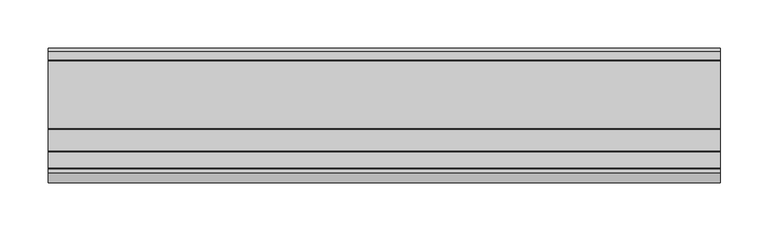
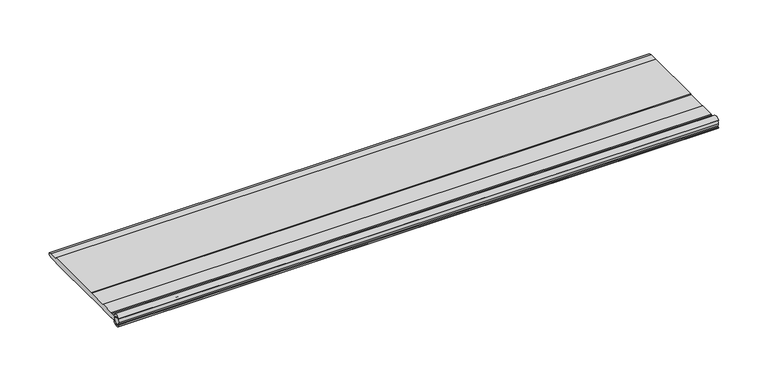
"""IFC4 building model written with IfcOpenShell, lengths in millimetres: proxy geometry, TN_Гидрошпонка ТН Фундамент : Гидрошпонка ТН Фундамент ТПС-В 140-1."""

import ifcopenshell
import ifcopenshell.guid

model = None  # the IFC model being written
_history = None  # IfcOwnerHistory: only IFC2X3 demands one
_inside = {}  # id of a spatial element -> (the spatial element, [elements in it])
_under = {}  # id of a project, library or spatial element -> (it, [spatial elements below it])
_declared = {}  # id of a project -> (the project, [libraries it declares])
_typed = {}  # id of a type object -> (the type object, [elements of that type])
_made_of = {}  # id of a material, layer set ... -> (it, [elements and type objects made of it])


def new_model(schema):
    """Start an empty IFC model of exactly this schema.

    Asked for "IFC4X3", IfcOpenShell would pick the latest addendum, in which some entities
    have other attributes; the version numbers below select the first issue.
    IFC2X3 requires an IfcOwnerHistory on every rooted entity: one is made here for all.
    """
    global model, _history
    if schema == "IFC4X3":
        model = ifcopenshell.file(schema_version=(4, 3, 0, 0))
    else:
        model = ifcopenshell.file(schema=schema)
    _inside.clear()
    _under.clear()
    _declared.clear()
    _typed.clear()
    _made_of.clear()
    _history = None
    if model.schema == "IFC2X3":
        org = make("IfcOrganization", Name="unknown")
        user = make(
            "IfcPersonAndOrganization",
            ThePerson=make("IfcPerson", FamilyName="unknown"),
            TheOrganization=org,
        )
        app = make(
            "IfcApplication",
            ApplicationDeveloper=org,
            Version="unknown",
            ApplicationFullName="unknown",
            ApplicationIdentifier="unknown",
        )
        _history = make(
            "IfcOwnerHistory",
            OwningUser=user,
            OwningApplication=app,
            ChangeAction="ADDED",
            CreationDate=0,
        )
    return model


def make(cls, **values):
    """One entity of the class cls with the attributes given. An attribute that is None is left unset."""
    return model.create_entity(
        cls, **{name: value for name, value in values.items() if value is not None}
    )


def rooted(cls, **values):
    """An entity with a GlobalId (a new one), such as an element, a storey or a relation."""
    return make(cls, GlobalId=ifcopenshell.guid.new(), OwnerHistory=_history, **values)


def si_unit(unit_type, name, prefix=None):
    """IfcSIUnit, for example si_unit("LENGTHUNIT", "METRE", prefix="MILLI")."""
    return make("IfcSIUnit", UnitType=unit_type, Prefix=prefix, Name=name)


def assignment(units):
    """IfcUnitAssignment: the units of a project."""
    return None if units is None else make("IfcUnitAssignment", Units=units)


def point(xyz):
    """IfcCartesianPoint."""
    return None if xyz is None else make("IfcCartesianPoint", Coordinates=xyz)


def direction(xyz):
    """IfcDirection."""
    return None if xyz is None else make("IfcDirection", DirectionRatios=xyz)


def frame(location, z_axis=None, x_axis=None):
    """IfcAxis2Placement3D, a coordinate frame: its origin and axes. An axis left out is left unset."""
    return make(
        "IfcAxis2Placement3D",
        Location=point(location),
        Axis=direction(z_axis),
        RefDirection=direction(x_axis),
    )


def frame_2d(location, x_axis=None):
    """IfcAxis2Placement2D, a coordinate frame in the plane: its origin and x axis."""
    return make(
        "IfcAxis2Placement2D", Location=point(location), RefDirection=direction(x_axis)
    )


def origin():
    """The frame at (0, 0, 0) with its axes left unset."""
    return frame((0.0, 0.0, 0.0))


def place(relative_to, where):
    """IfcLocalPlacement: puts the frame where relative to a parent placement (None: the world)."""
    return make(
        "IfcLocalPlacement", PlacementRelTo=relative_to, RelativePlacement=where
    )


def context(
    kind, dimensions, precision=None, world=None, true_north=None, identifier=None
):
    """IfcGeometricRepresentationContext, for example the 3D "Model" context."""
    return make(
        "IfcGeometricRepresentationContext",
        ContextIdentifier=identifier,
        ContextType=kind,
        CoordinateSpaceDimension=dimensions,
        Precision=precision,
        WorldCoordinateSystem=world,
        TrueNorth=true_north,
    )


def project(units=None, contexts=None):
    """IfcProject with its units and contexts."""
    return rooted(
        "IfcProject",
        Name="project",
        RepresentationContexts=contexts,
        UnitsInContext=assignment(units),
    )


def spatial(cls, under=None, at=None, **own):
    """A site, building, storey or space (cls), placed at a placement, below another one or the project."""
    s = rooted(cls, ObjectPlacement=at, **own)
    if under is not None:
        _under.setdefault(under.id(), (under, []))[1].append(s)
    return s


def polyline(points):
    """IfcPolyline through the points."""
    return make("IfcPolyline", Points=[point(p) for p in points])


def circle_curve(where, radius):
    """IfcCircle in the frame where."""
    return make("IfcCircle", Position=where, Radius=radius)


def trimmed(basis, trim1, trim2, sense, master):
    """IfcTrimmedCurve: the piece of a basis curve between two trims."""
    return make(
        "IfcTrimmedCurve",
        BasisCurve=basis,
        Trim1=trim1,
        Trim2=trim2,
        SenseAgreement=sense,
        MasterRepresentation=master,
    )


def segment(curve, same_sense, transition):
    """IfcCompositeCurveSegment."""
    return make(
        "IfcCompositeCurveSegment",
        Transition=transition,
        SameSense=same_sense,
        ParentCurve=curve,
    )


def composite_curve(segments, self_intersect=None):
    """IfcCompositeCurve: segments joined end to end."""
    return make("IfcCompositeCurve", Segments=segments, SelfIntersect=self_intersect)


def outline(outer, holes=None, kind="AREA"):
    """IfcArbitraryClosedProfileDef: a profile drawn as a closed curve; with holes, ...WithVoids."""
    if holes is None:
        return make("IfcArbitraryClosedProfileDef", ProfileType=kind, OuterCurve=outer)
    return make(
        "IfcArbitraryProfileDefWithVoids",
        ProfileType=kind,
        OuterCurve=outer,
        InnerCurves=holes,
    )


def extrude(swept, where, along, depth):
    """IfcExtrudedAreaSolid: the profile swept, set in the frame where, extruded along a direction by depth."""
    return make(
        "IfcExtrudedAreaSolid",
        SweptArea=swept,
        Position=where,
        ExtrudedDirection=direction(along),
        Depth=depth,
    )


def shape(context_of_items, identifier, shape_type, items):
    """IfcShapeRepresentation: the items that make up one representation, for example the "Body"."""
    return make(
        "IfcShapeRepresentation",
        ContextOfItems=context_of_items,
        RepresentationIdentifier=identifier,
        RepresentationType=shape_type,
        Items=items,
    )


def source(mapping_origin, context_of_items, identifier, shape_type, items):
    """IfcRepresentationMap: a shape defined once, which mapped items show again and again."""
    return make(
        "IfcRepresentationMap",
        MappingOrigin=mapping_origin,
        MappedRepresentation=shape(context_of_items, identifier, shape_type, items),
    )


def transform(
    local_origin,
    x_axis=None,
    y_axis=None,
    z_axis=None,
    scale=None,
    scale2=None,
    scale3=None,
    uniform=True,
):
    """IfcCartesianTransformationOperator3D, or its non-uniform kind. x_axis, y_axis, z_axis: its Axis1, 2, 3."""
    if uniform:
        return make(
            "IfcCartesianTransformationOperator3D",
            Axis1=direction(x_axis),
            Axis2=direction(y_axis),
            LocalOrigin=point(local_origin),
            Scale=scale,
            Axis3=direction(z_axis),
        )
    return make(
        "IfcCartesianTransformationOperator3DnonUniform",
        Axis1=direction(x_axis),
        Axis2=direction(y_axis),
        LocalOrigin=point(local_origin),
        Scale=scale,
        Axis3=direction(z_axis),
        Scale2=scale2,
        Scale3=scale3,
    )


def mapped(mapping_source, mapping_target):
    """IfcMappedItem: shows the shape of a source again, moved by a transform."""
    return make(
        "IfcMappedItem", MappingSource=mapping_source, MappingTarget=mapping_target
    )


def made_of(thing, what):
    """Note that an element or type object is made of a material, layer set ...; save() writes the relation."""
    if what is not None:
        _made_of.setdefault(what.id(), (what, []))[1].append(thing)
    return thing


def element(
    cls,
    number,
    at=None,
    inside=None,
    cuts=None,
    type_object=None,
    material=None,
    context=None,
    identifier="Body",
    shape_type=None,
    held_by="IfcProductDefinitionShape",
    body=None,
    shapes=None,
    **own,
):
    """One element of the class cls, such as IfcWall. Its Tag is "e" and its number.

    at: its placement. inside: the storey or other place that contains it. cuts: it is an
    opening in that element (IfcRelVoidsElement). A single representation is given by context,
    identifier, shape_type and body (its items); several are given by shapes. held_by: the class
    of the entity that holds the representations. save() writes the other relations.
    """
    e = rooted(cls, Tag="e%d" % number, ObjectPlacement=at, **own)
    if body is not None:
        shapes = [shape(context, identifier, shape_type, body)]
    if shapes is not None:
        e.Representation = make(held_by, Representations=shapes)
    if inside is not None:
        _inside.setdefault(inside.id(), (inside, []))[1].append(e)
    if cuts is not None:
        rooted(
            "IfcRelVoidsElement", RelatingBuildingElement=cuts, RelatedOpeningElement=e
        )
    if type_object is not None:
        _typed.setdefault(type_object.id(), (type_object, []))[1].append(e)
    return made_of(e, material)


def aggregate(whole, parts):
    """IfcRelAggregates: a whole, such as a stair, and the parts it consists of."""
    return rooted("IfcRelAggregates", RelatingObject=whole, RelatedObjects=parts)


def save(model, path):
    """Write the relations noted so far, then the file.

    IfcRelAggregates (storeys below a building ...), IfcRelContainedInSpatialStructure (elements
    in a storey), IfcRelDefinesByType, IfcRelAssociatesMaterial and IfcRelDeclares: one each for
    every whole, place, type object, material and project.
    """
    for whole, parts in _under.values():
        aggregate(whole, parts)
    for where, things in _inside.values():
        rooted(
            "IfcRelContainedInSpatialStructure",
            RelatedElements=things,
            RelatingStructure=where,
        )
    for kind, things in _typed.values():
        rooted("IfcRelDefinesByType", RelatedObjects=things, RelatingType=kind)
    for what, things in _made_of.values():
        rooted("IfcRelAssociatesMaterial", RelatedObjects=things, RelatingMaterial=what)
    for by, libraries in _declared.values():
        rooted("IfcRelDeclares", RelatingContext=by, RelatedDefinitions=libraries)
    model.write(path)


def specialty_equipment_85209dcb(model_context):
    return source(origin(), model_context, "Body", "SweptSolid", [
        extrude(outline(composite_curve([segment(trimmed(circle_curve(frame_2d((-66.1381773, 2.4826107)), 3.8618227), [point((-70.0, 2.4826107))], [point((-62.2763546, 2.4826107))], False, "CARTESIAN"), True, "CONTINUOUS"), segment(trimmed(circle_curve(frame_2d((-66.1381773, 2.4826107)), 3.8618227), [point((-62.2763546, 2.4826107))], [point((-70.0, 2.4826107))], False, "CARTESIAN"), True, "CONTINUOUS")], self_intersect=False)), frame((0.0, 0.0, 0.0), z_axis=(1.0, 0.0, 0.0), x_axis=(0.0, 1.0, 0.0)), (0.0, 0.0, 1.0), 700.0),
        extrude(outline(composite_curve([segment(polyline([(-60.205078, 5.0), (-56.0697209, 5.0), (-55.3626141, 5.7071068), (-38.3626141, 5.7071068), (-37.6555073, 5.0), (-15.0697209, 5.0), (-14.3626141, 5.7071068), (56.3972979, 5.7071068), (57.1044047, 5.0), (66.1226563, 5.0), (70.0, 3.9610689), (70.0, 1.0389311), (66.1226563, 0.0), (57.1044047, 0.0), (56.3652653, -0.7391394), (-14.3626141, -0.7391394), (-15.1017535, 0.0), (-37.6555073, 0.0), (-38.3946467, -0.7391394), (-55.3626141, -0.7391394), (-56.1017535, 0.0), (-60.1910456, 0.0)]), True, "CONTINUOUS"), segment(trimmed(circle_curve(frame_2d((-65.7633479, 1.0992351)), 5.6796893), [point((-60.1910456, 0.0))], [point((-70.267785, -2.3603771))], False, "CARTESIAN"), True, "CONTINUOUS"), segment(polyline([(-70.267785, -2.3603771), (-69.258949, -1.351541)]), True, "CONTINUOUS"), segment(trimmed(circle_curve(frame_2d((-66.1381773, 2.4826107)), 4.9436763), [point((-69.258949, -1.351541))], [point((-69.258949, 6.3167624))], True, "CARTESIAN"), True, "CONTINUOUS"), segment(polyline([(-69.258949, 6.3167624), (-70.2425291, 7.3003425)]), True, "CONTINUOUS"), segment(trimmed(circle_curve(frame_2d((-65.7633479, 3.7958916)), 5.6871997), [point((-70.2425291, 7.3003425))], [point((-60.205078, 5.0))], False, "CARTESIAN"), True, "CONTINUOUS")], self_intersect=False)), frame((0.0, 0.0, 0.0), z_axis=(1.0, 0.0, 0.0), x_axis=(0.0, 1.0, 0.0)), (0.0, 0.0, 1.0), 700.0),
    ])


if __name__ == "__main__":
    model = new_model("IFC4")
    model_context = context("Model", 3, world=origin())
    ifc_project = project(units=[si_unit("LENGTHUNIT", "METRE", prefix="MILLI")], contexts=[model_context])
    site = spatial("IfcSite", under=ifc_project)
    building = spatial("IfcBuilding", under=site)
    placement = place(None, origin())
    specialty_equipment_shape = specialty_equipment_85209dcb(model_context)
    element("IfcBuildingElementProxy", 1, Name="TN_Гидрошпонка ТН Фундамент : Гидрошпонка ТН Фундамент ТПС-В 140-1", ObjectType="TN_Гидрошпонка ТН Фундамент : Гидрошпонка ТН Фундамент ТПС-В 140-1", at=placement, inside=building, context=model_context, shape_type="MappedRepresentation", body=[
        mapped(specialty_equipment_shape, transform((0.0, 0.0, 0.0), x_axis=(1.0, 0.0, 0.0), y_axis=(0.0, 1.0, 0.0), z_axis=(0.0, 0.0, 1.0))),
    ])
    save(model, "model.ifc")

# Revit data of these elements
# Type "TN_Гидрошпонка ТН Фундамент : Гидрошпонка ТН Фундамент ТПС-В 140-1"
#   Description = "Внутренние гидроизоляционные шпонки ТН Фундамент ТПС-В предназначены для герметизации технологических швов бетонирования в местах сопряжения плиты и стены фундамента при строительстве подземных и заглубленных конструкций зданий и сооружений различного назначения и класса ответственности. Наличие набухающего шнура на краях шпонки позволяет повысить надежность шва."
#   Type Comments = "п.м."
#   Manufacturer = "ТехноНИКОЛЬ"
#   URL = "https://nav.tn.ru/catalog/gidroizolyatsiya/komplektatsiya-dlya-gidroizolyatsii/gidroshponki-tekhnonikol-fundament-tps-v/"
#   ADSK_Примечание = ""
#   ADSK_Обозначение [instance default] = "ТехноНИКОЛЬ"
#   ADSK_Наименование = "Гидрошпонка ТН Фундамент ТПС-В 140-1"
#   ADSK_Масса_Текст = ""
#   ADSK_Марка = ""
#   ADSK_Код изделия = "64369"
#   ADSK_Завод-изготовитель [instance default] = "ТехноНИКОЛЬ"
#   ADSK_Единица измерения [instance default] = "п.м."
#   ADSK_Группирование = "Гидрошпонки"
#   ADSK_URL страницы изделия = "https://nav.tn.ru/catalog/gidroizolyatsiya/komplektatsiya-dlya-gidroizolyatsii/gidroshponki-tekhnonikol-fundament-tps-v/"
#   ADSK_URL документации изделия = "https://nav.tn.ru/upload/iblock/39e/n34lwlimw5x5s3mf7b0hwzc10sm1ot3v/Tekhlist-7.400_Gidroshponki-TN-Fundament-TPS_V_RU_ru.pdf"
#   built-in parameter 1001306 [instance default] = 3.28084 (stored number, unit not read)
#   ADSK_Размер_Длина [instance default] = 1000 mm
#   ADSK_Количество [instance default] = 1
#   Гидрошпонка ТН Фундамент ТШ-Н-210 = no
#   Гидрошпонка ТН Фундамент ДШП-В-50 = no
#   Гидрошпонка ТН Фундамент ДШП-В-20 = no
#   Гидрошпонка ТН Фундамент ДШ-В-280 = no
#   Гидрошпонка ТН Фундамент ДШ-В-250 = no
#   Гидрошпонка ТН Фундамент ТШ-В-250 = no
#   Гидрошпонка ТН Фундамент ТПС-В 140-1 = yes
#   Гидрошпонка ТН Фундамент ДШ-Н-280 = no
#   Гидрошпонка ТН Фундамент ДШ-Н-250 = no
#   Гидрошпонка ТН Фундамент ТПС-В 100-2 = no
#   Гидрошпонка ТН Фундамент ТШ-Н-250 = no
#   Гидрошпонка ТН Фундамент ТШ-В-210 = no
#   Материал = TN_ПВХ_Черный
#   Default Elevation = 0
# Element 1 (IfcBuildingElementProxy, "TN_Гидрошпонка ТН Фундамент : Гидрошпонка ТН Фундамент ТПС-В 140-1")
#   built-in parameter 1001306 = 2.29659 (stored number, unit not read)
#   ADSK_Размер_Длина = 700 mm
#   ADSK_Количество = 0.7
#   Materials on its faces: "TN_ПВХ_Черный"
# Materials
#   "TN_ПВХ_Черный": class "Типовые", colour RGB 48 48 48, transparency 0, Cost = 0
